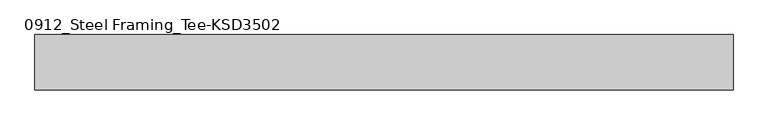
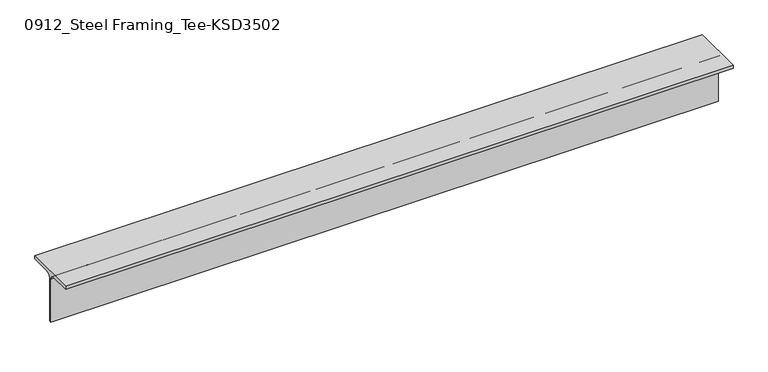
"""IFC4 building model written with IfcOpenShell, lengths in millimetres: member geometry, 0912_Steel Framing_Tee-KSD3502 : H_SB_ASB_CT-150x150x6.5x9."""

import ifcopenshell
import ifcopenshell.guid

model = None  # the IFC model being written
_history = None  # IfcOwnerHistory: only IFC2X3 demands one
_inside = {}  # id of a spatial element -> (the spatial element, [elements in it])
_under = {}  # id of a project, library or spatial element -> (it, [spatial elements below it])
_declared = {}  # id of a project -> (the project, [libraries it declares])
_typed = {}  # id of a type object -> (the type object, [elements of that type])
_made_of = {}  # id of a material, layer set ... -> (it, [elements and type objects made of it])


def new_model(schema):
    """Start an empty IFC model of exactly this schema.

    Asked for "IFC4X3", IfcOpenShell would pick the latest addendum, in which some entities
    have other attributes; the version numbers below select the first issue.
    IFC2X3 requires an IfcOwnerHistory on every rooted entity: one is made here for all.
    """
    global model, _history
    if schema == "IFC4X3":
        model = ifcopenshell.file(schema_version=(4, 3, 0, 0))
    else:
        model = ifcopenshell.file(schema=schema)
    _inside.clear()
    _under.clear()
    _declared.clear()
    _typed.clear()
    _made_of.clear()
    _history = None
    if model.schema == "IFC2X3":
        org = make("IfcOrganization", Name="unknown")
        user = make(
            "IfcPersonAndOrganization",
            ThePerson=make("IfcPerson", FamilyName="unknown"),
            TheOrganization=org,
        )
        app = make(
            "IfcApplication",
            ApplicationDeveloper=org,
            Version="unknown",
            ApplicationFullName="unknown",
            ApplicationIdentifier="unknown",
        )
        _history = make(
            "IfcOwnerHistory",
            OwningUser=user,
            OwningApplication=app,
            ChangeAction="ADDED",
            CreationDate=0,
        )
    return model


def make(cls, **values):
    """One entity of the class cls with the attributes given. An attribute that is None is left unset."""
    return model.create_entity(
        cls, **{name: value for name, value in values.items() if value is not None}
    )


def rooted(cls, **values):
    """An entity with a GlobalId (a new one), such as an element, a storey or a relation."""
    return make(cls, GlobalId=ifcopenshell.guid.new(), OwnerHistory=_history, **values)


def si_unit(unit_type, name, prefix=None):
    """IfcSIUnit, for example si_unit("LENGTHUNIT", "METRE", prefix="MILLI")."""
    return make("IfcSIUnit", UnitType=unit_type, Prefix=prefix, Name=name)


def assignment(units):
    """IfcUnitAssignment: the units of a project."""
    return None if units is None else make("IfcUnitAssignment", Units=units)


def point(xyz):
    """IfcCartesianPoint."""
    return None if xyz is None else make("IfcCartesianPoint", Coordinates=xyz)


def direction(xyz):
    """IfcDirection."""
    return None if xyz is None else make("IfcDirection", DirectionRatios=xyz)


def frame(location, z_axis=None, x_axis=None):
    """IfcAxis2Placement3D, a coordinate frame: its origin and axes. An axis left out is left unset."""
    return make(
        "IfcAxis2Placement3D",
        Location=point(location),
        Axis=direction(z_axis),
        RefDirection=direction(x_axis),
    )


def frame_2d(location, x_axis=None):
    """IfcAxis2Placement2D, a coordinate frame in the plane: its origin and x axis."""
    return make(
        "IfcAxis2Placement2D", Location=point(location), RefDirection=direction(x_axis)
    )


def origin():
    """The frame at (0, 0, 0) with its axes left unset."""
    return frame((0.0, 0.0, 0.0))


def place(relative_to, where):
    """IfcLocalPlacement: puts the frame where relative to a parent placement (None: the world)."""
    return make(
        "IfcLocalPlacement", PlacementRelTo=relative_to, RelativePlacement=where
    )


def context(
    kind, dimensions, precision=None, world=None, true_north=None, identifier=None
):
    """IfcGeometricRepresentationContext, for example the 3D "Model" context."""
    return make(
        "IfcGeometricRepresentationContext",
        ContextIdentifier=identifier,
        ContextType=kind,
        CoordinateSpaceDimension=dimensions,
        Precision=precision,
        WorldCoordinateSystem=world,
        TrueNorth=true_north,
    )


def project(units=None, contexts=None):
    """IfcProject with its units and contexts."""
    return rooted(
        "IfcProject",
        Name="project",
        RepresentationContexts=contexts,
        UnitsInContext=assignment(units),
    )


def spatial(cls, under=None, at=None, **own):
    """A site, building, storey or space (cls), placed at a placement, below another one or the project."""
    s = rooted(cls, ObjectPlacement=at, **own)
    if under is not None:
        _under.setdefault(under.id(), (under, []))[1].append(s)
    return s


def polyline(points):
    """IfcPolyline through the points."""
    return make("IfcPolyline", Points=[point(p) for p in points])


def circle_curve(where, radius):
    """IfcCircle in the frame where."""
    return make("IfcCircle", Position=where, Radius=radius)


def trimmed(basis, trim1, trim2, sense, master):
    """IfcTrimmedCurve: the piece of a basis curve between two trims."""
    return make(
        "IfcTrimmedCurve",
        BasisCurve=basis,
        Trim1=trim1,
        Trim2=trim2,
        SenseAgreement=sense,
        MasterRepresentation=master,
    )


def segment(curve, same_sense, transition):
    """IfcCompositeCurveSegment."""
    return make(
        "IfcCompositeCurveSegment",
        Transition=transition,
        SameSense=same_sense,
        ParentCurve=curve,
    )


def composite_curve(segments, self_intersect=None):
    """IfcCompositeCurve: segments joined end to end."""
    return make("IfcCompositeCurve", Segments=segments, SelfIntersect=self_intersect)


def outline(outer, holes=None, kind="AREA"):
    """IfcArbitraryClosedProfileDef: a profile drawn as a closed curve; with holes, ...WithVoids."""
    if holes is None:
        return make("IfcArbitraryClosedProfileDef", ProfileType=kind, OuterCurve=outer)
    return make(
        "IfcArbitraryProfileDefWithVoids",
        ProfileType=kind,
        OuterCurve=outer,
        InnerCurves=holes,
    )


def extrude(swept, where, along, depth):
    """IfcExtrudedAreaSolid: the profile swept, set in the frame where, extruded along a direction by depth."""
    return make(
        "IfcExtrudedAreaSolid",
        SweptArea=swept,
        Position=where,
        ExtrudedDirection=direction(along),
        Depth=depth,
    )


def shape(context_of_items, identifier, shape_type, items):
    """IfcShapeRepresentation: the items that make up one representation, for example the "Body"."""
    return make(
        "IfcShapeRepresentation",
        ContextOfItems=context_of_items,
        RepresentationIdentifier=identifier,
        RepresentationType=shape_type,
        Items=items,
    )


def source(mapping_origin, context_of_items, identifier, shape_type, items):
    """IfcRepresentationMap: a shape defined once, which mapped items show again and again."""
    return make(
        "IfcRepresentationMap",
        MappingOrigin=mapping_origin,
        MappedRepresentation=shape(context_of_items, identifier, shape_type, items),
    )


def transform(
    local_origin,
    x_axis=None,
    y_axis=None,
    z_axis=None,
    scale=None,
    scale2=None,
    scale3=None,
    uniform=True,
):
    """IfcCartesianTransformationOperator3D, or its non-uniform kind. x_axis, y_axis, z_axis: its Axis1, 2, 3."""
    if uniform:
        return make(
            "IfcCartesianTransformationOperator3D",
            Axis1=direction(x_axis),
            Axis2=direction(y_axis),
            LocalOrigin=point(local_origin),
            Scale=scale,
            Axis3=direction(z_axis),
        )
    return make(
        "IfcCartesianTransformationOperator3DnonUniform",
        Axis1=direction(x_axis),
        Axis2=direction(y_axis),
        LocalOrigin=point(local_origin),
        Scale=scale,
        Axis3=direction(z_axis),
        Scale2=scale2,
        Scale3=scale3,
    )


def mapped(mapping_source, mapping_target):
    """IfcMappedItem: shows the shape of a source again, moved by a transform."""
    return make(
        "IfcMappedItem", MappingSource=mapping_source, MappingTarget=mapping_target
    )


def made_of(thing, what):
    """Note that an element or type object is made of a material, layer set ...; save() writes the relation."""
    if what is not None:
        _made_of.setdefault(what.id(), (what, []))[1].append(thing)
    return thing


def element(
    cls,
    number,
    at=None,
    inside=None,
    cuts=None,
    type_object=None,
    material=None,
    context=None,
    identifier="Body",
    shape_type=None,
    held_by="IfcProductDefinitionShape",
    body=None,
    shapes=None,
    **own,
):
    """One element of the class cls, such as IfcWall. Its Tag is "e" and its number.

    at: its placement. inside: the storey or other place that contains it. cuts: it is an
    opening in that element (IfcRelVoidsElement). A single representation is given by context,
    identifier, shape_type and body (its items); several are given by shapes. held_by: the class
    of the entity that holds the representations. save() writes the other relations.
    """
    e = rooted(cls, Tag="e%d" % number, ObjectPlacement=at, **own)
    if body is not None:
        shapes = [shape(context, identifier, shape_type, body)]
    if shapes is not None:
        e.Representation = make(held_by, Representations=shapes)
    if inside is not None:
        _inside.setdefault(inside.id(), (inside, []))[1].append(e)
    if cuts is not None:
        rooted(
            "IfcRelVoidsElement", RelatingBuildingElement=cuts, RelatedOpeningElement=e
        )
    if type_object is not None:
        _typed.setdefault(type_object.id(), (type_object, []))[1].append(e)
    return made_of(e, material)


def aggregate(whole, parts):
    """IfcRelAggregates: a whole, such as a stair, and the parts it consists of."""
    return rooted("IfcRelAggregates", RelatingObject=whole, RelatedObjects=parts)


def save(model, path):
    """Write the relations noted so far, then the file.

    IfcRelAggregates (storeys below a building ...), IfcRelContainedInSpatialStructure (elements
    in a storey), IfcRelDefinesByType, IfcRelAssociatesMaterial and IfcRelDeclares: one each for
    every whole, place, type object, material and project.
    """
    for whole, parts in _under.values():
        aggregate(whole, parts)
    for where, things in _inside.values():
        rooted(
            "IfcRelContainedInSpatialStructure",
            RelatedElements=things,
            RelatingStructure=where,
        )
    for kind, things in _typed.values():
        rooted("IfcRelDefinesByType", RelatedObjects=things, RelatingType=kind)
    for what, things in _made_of.values():
        rooted("IfcRelAssociatesMaterial", RelatedObjects=things, RelatingMaterial=what)
    for by, libraries in _declared.values():
        rooted("IfcRelDeclares", RelatingContext=by, RelatedDefinitions=libraries)
    model.write(path)


def member_0912_steel_framing_tee_ksd3502_bb1c0123(model_context):
    return source(origin(), model_context, "Body", "SweptSolid", [
        extrude(outline(composite_curve([segment(polyline([(75.0, 75.0), (75.0, 66.0), (16.25, 66.0)]), True, "CONTINUOUS"), segment(trimmed(circle_curve(frame_2d((16.25, 53.0)), 13.0), [point((16.25, 66.0))], [point((3.25, 53.0))], True, "CARTESIAN"), True, "CONTINUOUS"), segment(polyline([(3.25, 53.0), (3.25, -75.0), (-3.25, -75.0), (-3.25, 53.0)]), True, "CONTINUOUS"), segment(trimmed(circle_curve(frame_2d((-16.25, 53.0)), 13.0), [point((-3.25, 53.0))], [point((-16.25, 66.0))], True, "CARTESIAN"), True, "CONTINUOUS"), segment(polyline([(-16.25, 66.0), (-75.0, 66.0), (-75.0, 75.0), (75.0, 75.0)]), True, "CONTINUOUS")], self_intersect=False)), frame((-900.05, 0.0, 0.0), z_axis=(1.0, 0.0, 0.0), x_axis=(0.0, 1.0, 0.0)), (0.0, 0.0, 1.0), 1884.0),
    ])


if __name__ == "__main__":
    model = new_model("IFC4")
    model_context = context("Model", 3, world=origin())
    ifc_project = project(units=[si_unit("LENGTHUNIT", "METRE", prefix="MILLI")], contexts=[model_context])
    site = spatial("IfcSite", under=ifc_project)
    building = spatial("IfcBuilding", under=site)
    placement = place(None, origin())
    member_0912_steel_framing_tee_ksd3502_shape = member_0912_steel_framing_tee_ksd3502_bb1c0123(model_context)
    element("IfcMember", 1, ObjectType="0912_Steel Framing_Tee-KSD3502 : H_SB_ASB_CT-150x150x6.5x9", at=placement, inside=building, context=model_context, shape_type="MappedRepresentation", body=[
        mapped(member_0912_steel_framing_tee_ksd3502_shape, transform((0.0, 0.0, 0.0), x_axis=(1.0, 0.0, 0.0), y_axis=(0.0, 1.0, 0.0), z_axis=(0.0, 0.0, 1.0))),
    ])
    save(model, "model.ifc")

# Revit data of these elements
# Type "0912_Steel Framing_Tee-KSD3502 : H_SB_ASB_CT-150x150x6.5x9"
#   H_WM Code_1 = "S01AA003-00001 | Main Steel Structure Fabrication Work | Shelter/Building | Light Steel - Standard (30KG/M>Weight) | Material: (   )"
#   H_WM Code_2 = "S03AA029-00001 | Main Steel Structure Erection Work | Shelter/Building | Light Steel (30KG/M>Weight) | Material: (   )"
#   H_WM Code_3 = "S01AA010-00001 | Main Steel Structure Fabrication Work | Shelter/Building | Steel Painting/Coating | for Non-Fireproofed Steel Surface, Surface Preparation, Primer, Second & Final Coat | Material: (   )"
#   H_Q'ty Cal Type Tag = "SB-Q2"
#   Width = 15.0 cm
#   Web Thickness = 0.65 cm
#   Web Fillet = 1.3 cm
#   Section Area = 23.39 cm²
#   Perimeter = 0.60 m²/m
#   Nominal Weight = 18.40 kgf/m
#   Height = 15.0 cm
#   Flange Thickness = 0.9 cm
#   Centroid Vertical = 7.5 cm
#   Centroid Horizontal = 7.5 cm
#   Length [instance default] = 1.5000 m
#   Structural Material [instance default] = Steel, 45-345
#   Warping Constant = (empty or 0)
#   Torsional Moment of Inertia = 0
#   Section Name Key = ""
#   Plastic Modulus weak axis = 0
#   Plastic Modulus strong axis = 0
#   Moment of Inertia weak axis = 0
#   Moment of Inertia strong axis = 0
#   Elastic Modulus weak axis = 0
#   Elastic Modulus strong axis = 0
#   Bolt Spacing = 0
#   Assembly Code = ""
# Element 1 (IfcMember, "0912_Steel Framing_Tee-KSD3502 : H_SB_ASB_CT-150x150x6.5x9")
#   Structural Material = none
# Materials
#   "Steel, 45-345": class "Metal", colour RGB 189 187 185, transparency 0, Description = "Steel 345 MPa", Cost = 0
